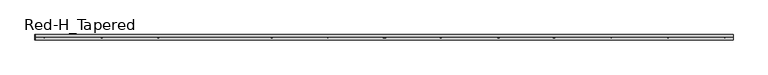
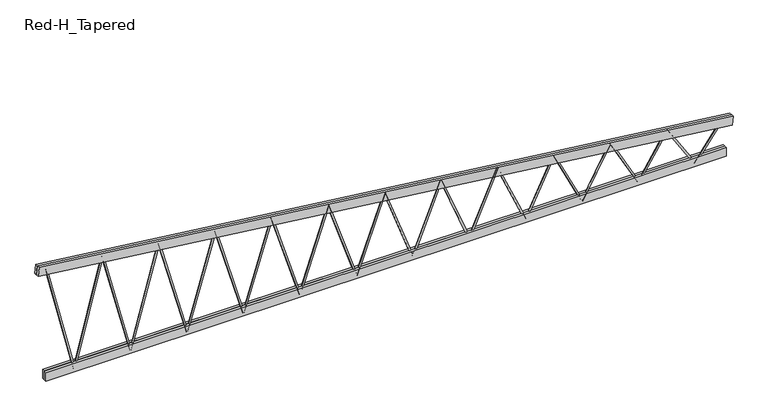
"""IFC4 building model written with IfcOpenShell, lengths in millimetres: beam geometry, Construction_Frames_RedBuilt_Openweb_Red-H_Tapered : Red-H_Tapered."""

from ifc_helpers import new_model, si_unit, point, frame, origin, origin_2d, place, context, project, spatial, polyline, circle_curve, trimmed, segment, composite_curve, outline, extrude, source, transform, mapped, element, save


def red_h_tapered_3554e35e(model_context):
    return source(origin(), model_context, "Body", "SweptSolid", [
        extrude(outline(composite_curve([segment(trimmed(circle_curve(origin_2d(), 12.7), [point((0.0, -12.7))], [point((0.0, 12.7))], False, "CARTESIAN"), True, "CONTINUOUS"), segment(trimmed(circle_curve(origin_2d(), 12.7), [point((0.0, 12.7))], [point((0.0, -12.7))], False, "CARTESIAN"), True, "CONTINUOUS")], self_intersect=False)), frame((-430.2126756, 0.0, -367.0101562), z_axis=(-0.31873146739711766, 0.0, 0.9478450567950861), x_axis=(0.0, -1.0, 0.0)), (0.0, 0.0, 1.0), 1349.7653027),
        extrude(outline(composite_curve([segment(trimmed(circle_curve(origin_2d(), 12.7), [point((0.0, 12.7))], [point((0.0, -12.7))], False, "CARTESIAN"), True, "CONTINUOUS"), segment(trimmed(circle_curve(origin_2d(), 12.7), [point((0.0, -12.7))], [point((0.0, 12.7))], False, "CARTESIAN"), True, "CONTINUOUS")], self_intersect=False)), frame((-1290.6380267, 0.0, -367.0101562), z_axis=(0.3187314673971197, 0.0, 0.9478450567950856), x_axis=(0.0, -1.0, 0.0)), (0.0, 0.0, 1.0), 1349.7653027),
        extrude(outline(composite_curve([segment(trimmed(circle_curve(origin_2d(), 12.7), [point((0.0, -12.7))], [point((0.0, 12.7))], False, "CARTESIAN"), True, "CONTINUOUS"), segment(trimmed(circle_curve(origin_2d(), 12.7), [point((0.0, 12.7))], [point((0.0, -12.7))], False, "CARTESIAN"), True, "CONTINUOUS")], self_intersect=False)), frame((-1290.6380267, 0.0, -367.0101562), z_axis=(-0.2978811940467248, 0.0, 0.954602951091865), x_axis=(0.0, -1.0, 0.0)), (0.0, 0.0, 1.0), 1444.2424838),
        extrude(outline(composite_curve([segment(trimmed(circle_curve(origin_2d(), 12.7), [point((0.0, -12.6999999))], [point((0.0, 12.7))], False, "CARTESIAN"), True, "CONTINUOUS"), segment(trimmed(circle_curve(origin_2d(), 12.7), [point((0.0, 12.7))], [point((0.0, -12.6999999))], False, "CARTESIAN"), True, "CONTINUOUS")], self_intersect=False)), frame((-2151.0633779, 0.0, -367.0101562), z_axis=(0.29788119404672875, 0.0, 0.9546029510918638), x_axis=(0.0, -1.0, 0.0)), (0.0, 0.0, 1.0), 1444.2424838),
        extrude(outline(composite_curve([segment(trimmed(circle_curve(origin_2d(), 12.7), [point((0.0, 12.7))], [point((0.0, -12.7))], False, "CARTESIAN"), True, "CONTINUOUS"), segment(trimmed(circle_curve(origin_2d(), 12.7), [point((0.0, -12.7))], [point((0.0, 12.7))], False, "CARTESIAN"), True, "CONTINUOUS")], self_intersect=False)), frame((-2151.0633779, 0.0, -367.0101562), z_axis=(-0.27948080603698605, 0.0, 0.9601512792559913), x_axis=(0.0, -1.0, 0.0)), (0.0, 0.0, 1.0), 1539.3281624),
        extrude(outline(composite_curve([segment(trimmed(circle_curve(origin_2d(), 12.7), [point((0.0, -12.6999999))], [point((0.0, 12.7))], False, "CARTESIAN"), True, "CONTINUOUS"), segment(trimmed(circle_curve(origin_2d(), 12.7), [point((0.0, 12.7))], [point((0.0, -12.6999999))], False, "CARTESIAN"), True, "CONTINUOUS")], self_intersect=False)), frame((-3011.488729, 0.0, -367.0101562), z_axis=(0.2794808060369842, 0.0, 0.9601512792559919), x_axis=(0.0, -1.0, 0.0)), (0.0, 0.0, 1.0), 1539.3281624),
        extrude(outline(composite_curve([segment(trimmed(circle_curve(origin_2d(), 12.7), [point((0.0, 12.7))], [point((0.0, -12.7))], False, "CARTESIAN"), True, "CONTINUOUS"), segment(trimmed(circle_curve(origin_2d(), 12.7), [point((0.0, -12.7))], [point((0.0, 12.7))], False, "CARTESIAN"), True, "CONTINUOUS")], self_intersect=False)), frame((-3011.488729, 0.0, -367.0101562), z_axis=(-0.2631405101102769, 0.0, 0.9647575197628175), x_axis=(0.0, -1.0, 0.0)), (0.0, 0.0, 1.0), 1634.9161723),
        extrude(outline(composite_curve([segment(trimmed(circle_curve(origin_2d(), 12.7), [point((0.0, -12.7))], [point((0.0, 12.7))], False, "CARTESIAN"), True, "CONTINUOUS"), segment(trimmed(circle_curve(origin_2d(), 12.7), [point((0.0, 12.7))], [point((0.0, -12.7))], False, "CARTESIAN"), True, "CONTINUOUS")], self_intersect=False)), frame((-3871.9140801, 0.0, -367.0101562), z_axis=(0.26314051011028217, 0.0, 0.9647575197628161), x_axis=(0.0, -1.0, 0.0)), (0.0, 0.0, 1.0), 1634.9161723),
        extrude(outline(composite_curve([segment(trimmed(circle_curve(origin_2d(), 12.7), [point((0.0, 12.7))], [point((0.0, -12.7))], False, "CARTESIAN"), True, "CONTINUOUS"), segment(trimmed(circle_curve(origin_2d(), 12.7), [point((0.0, -12.7))], [point((0.0, 12.7))], False, "CARTESIAN"), True, "CONTINUOUS")], self_intersect=False)), frame((-3871.9140801, 0.0, -367.0101562), z_axis=(-0.2485451996014145, 0.0, 0.9686202990620696), x_axis=(0.0, -1.0, 0.0)), (0.0, 0.0, 1.0), 1730.9232939),
        extrude(outline(composite_curve([segment(trimmed(circle_curve(origin_2d(), 12.7), [point((0.0, -12.7))], [point((0.0, 12.7))], False, "CARTESIAN"), True, "CONTINUOUS"), segment(trimmed(circle_curve(origin_2d(), 12.7), [point((0.0, 12.7))], [point((0.0, -12.7))], False, "CARTESIAN"), True, "CONTINUOUS")], self_intersect=False)), frame((-4732.3394313, 0.0, -367.0101562), z_axis=(0.24854519960141414, 0.0, 0.9686202990620696), x_axis=(0.0, -1.0, 0.0)), (0.0, 0.0, 1.0), 1730.9232939),
        extrude(outline(composite_curve([segment(trimmed(circle_curve(origin_2d(), 12.7), [point((0.0, 12.7))], [point((0.0, -12.7))], False, "CARTESIAN"), True, "CONTINUOUS"), segment(trimmed(circle_curve(origin_2d(), 12.7), [point((0.0, -12.7))], [point((0.0, 12.7))], False, "CARTESIAN"), True, "CONTINUOUS")], self_intersect=False)), frame((-4732.3394313, 0.0, -367.0101562), z_axis=(-0.2354383889559608, 0.0, 0.9718892761039303), x_axis=(0.0, -1.0, 0.0)), (0.0, 0.0, 1.0), 1827.2834667),
        extrude(outline(composite_curve([segment(trimmed(circle_curve(origin_2d(), 12.7), [point((0.0, 12.7000001))], [point((0.0, -12.7))], False, "CARTESIAN"), True, "CONTINUOUS"), segment(trimmed(circle_curve(origin_2d(), 12.7), [point((0.0, -12.7))], [point((0.0, 12.7000001))], False, "CARTESIAN"), True, "CONTINUOUS")], self_intersect=False)), frame((4732.3394313, 0.0, -367.0101562), z_axis=(0.5929752551345785, 0.0, 0.8052206820481461), x_axis=(0.0, -1.0, 0.0)), (0.0, 0.0, 1.0), 725.5153935),
        extrude(outline(composite_curve([segment(trimmed(circle_curve(origin_2d(), 12.7), [point((0.0, -12.7))], [point((0.0, 12.6999999))], False, "CARTESIAN"), True, "CONTINUOUS"), segment(trimmed(circle_curve(origin_2d(), 12.7), [point((0.0, 12.6999999))], [point((0.0, -12.7))], False, "CARTESIAN"), True, "CONTINUOUS")], self_intersect=False)), frame((4732.3394313, 0.0, -367.0101562), z_axis=(-0.5326844059976107, 0.0, 0.8463139627862539), x_axis=(0.0, -1.0, 0.0)), (0.0, 0.0, 1.0), 807.6314432),
        extrude(outline(composite_curve([segment(trimmed(circle_curve(origin_2d(), 12.7), [point((0.0, 12.7000001))], [point((0.0, -12.6999999))], False, "CARTESIAN"), True, "CONTINUOUS"), segment(trimmed(circle_curve(origin_2d(), 12.7), [point((0.0, -12.6999999))], [point((0.0, 12.7000001))], False, "CARTESIAN"), True, "CONTINUOUS")], self_intersect=False)), frame((3871.9140801, 0.0, -367.0101562), z_axis=(0.5326844059976091, 0.0, 0.8463139627862549), x_axis=(0.0, -1.0, 0.0)), (0.0, 0.0, 1.0), 807.6314432),
        extrude(outline(composite_curve([segment(trimmed(circle_curve(origin_2d(), 12.7), [point((0.0, -12.7))], [point((0.0, 12.7))], False, "CARTESIAN"), True, "CONTINUOUS"), segment(trimmed(circle_curve(origin_2d(), 12.7), [point((0.0, 12.7))], [point((0.0, -12.7))], False, "CARTESIAN"), True, "CONTINUOUS")], self_intersect=False)), frame((3871.9140801, 0.0, -367.0101562), z_axis=(-0.4816281502046464, 0.0, 0.8763756756839219), x_axis=(0.0, -1.0, 0.0)), (0.0, 0.0, 1.0), 893.2465334),
        extrude(outline(composite_curve([segment(trimmed(circle_curve(origin_2d(), 12.7), [point((0.0, 12.7000001))], [point((0.0, -12.7))], False, "CARTESIAN"), True, "CONTINUOUS"), segment(trimmed(circle_curve(origin_2d(), 12.7), [point((0.0, -12.7))], [point((0.0, 12.7000001))], False, "CARTESIAN"), True, "CONTINUOUS")], self_intersect=False)), frame((3011.488729, 0.0, -367.0101562), z_axis=(0.48162815020464855, 0.0, 0.8763756756839207), x_axis=(0.0, -1.0, 0.0)), (0.0, 0.0, 1.0), 893.2465334),
        extrude(outline(composite_curve([segment(trimmed(circle_curve(origin_2d(), 12.7), [point((0.0, -12.7))], [point((0.0, 12.7))], False, "CARTESIAN"), True, "CONTINUOUS"), segment(trimmed(circle_curve(origin_2d(), 12.7), [point((0.0, 12.7))], [point((0.0, -12.7))], False, "CARTESIAN"), True, "CONTINUOUS")], self_intersect=False)), frame((3011.488729, 0.0, -367.0101562), z_axis=(-0.43834601558162534, 0.0, 0.8988063031731105), x_axis=(0.0, -1.0, 0.0)), (0.0, 0.0, 1.0), 981.4453885),
        extrude(outline(composite_curve([segment(trimmed(circle_curve(origin_2d(), 12.7), [point((0.0, 12.7))], [point((0.0, -12.7))], False, "CARTESIAN"), True, "CONTINUOUS"), segment(trimmed(circle_curve(origin_2d(), 12.7), [point((0.0, -12.7))], [point((0.0, 12.7))], False, "CARTESIAN"), True, "CONTINUOUS")], self_intersect=False)), frame((2151.0633779, 0.0, -367.0101562), z_axis=(0.43834601558162795, 0.0, 0.8988063031731094), x_axis=(0.0, -1.0, 0.0)), (0.0, 0.0, 1.0), 981.4453885),
        extrude(outline(composite_curve([segment(trimmed(circle_curve(origin_2d(), 12.7), [point((0.0, -12.7))], [point((0.0, 12.6999999))], False, "CARTESIAN"), True, "CONTINUOUS"), segment(trimmed(circle_curve(origin_2d(), 12.7), [point((0.0, 12.6999999))], [point((0.0, -12.7))], False, "CARTESIAN"), True, "CONTINUOUS")], self_intersect=False)), frame((2151.0633779, 0.0, -367.0101562), z_axis=(-0.4014712611706427, 0.0, 0.9158716211642621), x_axis=(0.0, -1.0, 0.0)), (0.0, 0.0, 1.0), 1071.5902162),
        extrude(outline(composite_curve([segment(trimmed(circle_curve(origin_2d(), 12.7), [point((0.0, 12.7))], [point((0.0, -12.7))], False, "CARTESIAN"), True, "CONTINUOUS"), segment(trimmed(circle_curve(origin_2d(), 12.7), [point((0.0, -12.7))], [point((0.0, 12.7))], False, "CARTESIAN"), True, "CONTINUOUS")], self_intersect=False)), frame((1290.6380267, 0.0, -367.0101562), z_axis=(0.4014712611706487, 0.0, 0.9158716211642596), x_axis=(0.0, -1.0, 0.0)), (0.0, 0.0, 1.0), 1071.5902162),
        extrude(outline(composite_curve([segment(trimmed(circle_curve(origin_2d(), 12.7), [point((0.0, -12.7))], [point((0.0, 12.7))], False, "CARTESIAN"), True, "CONTINUOUS"), segment(trimmed(circle_curve(origin_2d(), 12.7), [point((0.0, 12.7))], [point((0.0, -12.7))], False, "CARTESIAN"), True, "CONTINUOUS")], self_intersect=False)), frame((1290.6380267, 0.0, -367.0101562), z_axis=(-0.36984358980866666, 0.0, 0.9290940313431353), x_axis=(0.0, -1.0, 0.0)), (0.0, 0.0, 1.0), 1163.228693),
        extrude(outline(composite_curve([segment(trimmed(circle_curve(origin_2d(), 12.7), [point((0.0, 12.7))], [point((0.0, -12.7))], False, "CARTESIAN"), True, "CONTINUOUS"), segment(trimmed(circle_curve(origin_2d(), 12.7), [point((0.0, -12.7))], [point((0.0, 12.7))], False, "CARTESIAN"), True, "CONTINUOUS")], self_intersect=False)), frame((430.2126756, 0.0, -367.0101562), z_axis=(0.3698435898086691, 0.0, 0.9290940313431343), x_axis=(0.0, -1.0, 0.0)), (0.0, 0.0, 1.0), 1163.228693),
        extrude(outline(composite_curve([segment(trimmed(circle_curve(origin_2d(), 12.7), [point((0.0, -12.7))], [point((0.0, 12.7))], False, "CARTESIAN"), True, "CONTINUOUS"), segment(trimmed(circle_curve(origin_2d(), 12.7), [point((0.0, 12.7))], [point((0.0, -12.7))], False, "CARTESIAN"), True, "CONTINUOUS")], self_intersect=False)), frame((430.2126756, 0.0, -367.0101562), z_axis=(-0.3425167606493955, 0.0, 0.9395117182208239), x_axis=(0.0, -1.0, 0.0)), (0.0, 0.0, 1.0), 1256.0339376),
        extrude(outline(composite_curve([segment(trimmed(circle_curve(origin_2d(), 12.7), [point((0.0, 12.7))], [point((0.0, -12.7))], False, "CARTESIAN"), True, "CONTINUOUS"), segment(trimmed(circle_curve(origin_2d(), 12.7), [point((0.0, -12.7))], [point((0.0, 12.7))], False, "CARTESIAN"), True, "CONTINUOUS")], self_intersect=False)), frame((-430.2126756, 0.0, -367.0101562), z_axis=(0.3425167606493624, 0.0, 0.9395117182208359), x_axis=(0.0, -1.0, 0.0)), (0.0, 0.0, 1.0), 1256.0339376),
        extrude(outline(polyline([(-5187.9521069, -41.275), (-5187.9521069, -3.175), (5187.9521069, -3.175), (5187.9521069, -41.275), (-5187.9521069, -41.275)])), frame((0.0, 0.0, -386.0601562), z_axis=(0.0, 0.0, 1.0), x_axis=(1.0, 0.0, 0.0)), (0.0, 0.0, 1.0), 139.7),
        extrude(outline(polyline([(-5187.9521069, 3.175), (-5187.9521069, 41.275), (5187.9521069, 41.275), (5187.9521069, 3.175), (-5187.9521069, 3.175)])), frame((0.0, 0.0, -386.0601562), z_axis=(0.0, 0.0, 1.0), x_axis=(1.0, 0.0, 0.0)), (0.0, 0.0, 1.0), 139.7),
        extrude(outline(polyline([(0.0, -38.1), (0.0, 0.0), (10654.1188147, 0.0), (10654.1188147, -38.1), (0.0, -38.1)])), frame((-5306.1006487, -3.175, 1346.8859577), z_axis=(0.11845770841726733, 0.0, 0.9929590985113786), x_axis=(0.9929590985113786, 0.0, -0.11845770841726733)), (0.0, 0.0, 1.0), 139.7),
        extrude(outline(polyline([(0.0, -38.1), (0.0, 0.0), (10654.1188147, 0.0), (10654.1188147, -38.1), (0.0, -38.1)])), frame((-5306.1006487, 41.275, 1346.8859577), z_axis=(0.11845770841726733, 0.0, 0.9929590985113786), x_axis=(0.9929590985113786, 0.0, -0.11845770841726733)), (0.0, 0.0, 1.0), 139.7),
    ])


if __name__ == "__main__":
    model = new_model("IFC4")
    model_context = context("Model", 3, world=origin())
    ifc_project = project(units=[si_unit("LENGTHUNIT", "METRE", prefix="MILLI")], contexts=[model_context])
    site = spatial("IfcSite", under=ifc_project)
    building = spatial("IfcBuilding", under=site)
    placement = place(None, origin())
    red_h_tapered_shape = red_h_tapered_3554e35e(model_context)
    element("IfcBeam", 1, ObjectType="Construction_Frames_RedBuilt_Openweb_Red-H_Tapered : Red-H_Tapered", at=placement, inside=building, context=model_context, shape_type="MappedRepresentation", body=[
        mapped(red_h_tapered_shape, transform((0.0, 0.0, 0.0), x_axis=(1.0, 0.0, 0.0), y_axis=(0.0, 1.0, 0.0), z_axis=(0.0, 0.0, 1.0))),
    ])
    save(model, "model.ifc")

# Revit data of these elements
# Type "Construction_Frames_RedBuilt_Openweb_Red-H_Tapered : Red-H_Tapered"
#   Youtube clip = ""
#   Weight Net (Kg) = "0"
#   Webs = "Up to 2\" diameter tubular steel"
#   Uniformat II Description = ""
#   Uniformat II Code = ""
#   Uniclass 2015 Name = "Softwood trusses"
#   Uniclass 2015 Code = "Pr_20_85_90_81"
#   Uniclass 2.0 Description = "Structural Framing Systems"
#   Uniclass 2.0 Code = "SS-15-10-75"
#   Uniclass 1.4 Description = "Trusses"
#   Uniclass 1.4 Code = "L3523"
#   UNSPSC Code = "30103606"
#   Technical description = "http://www.redbuilt.com/reference/literature-and-other-resources"
#   Region South America = "None"
#   Region Oceania = "None"
#   Region North America = "US"
#   Region Middle East = "None"
#   Region Europe = "None"
#   Region Asia = "None"
#   Region Antarctica = "None"
#   Region Africa = "None"
#   QR code = "http://bimobject.com/redbuilt/product/redbuilt-0003"
#   Product url = "http://www.redbuilt.com/products/default.aspx?id=2"
#   Product group = "Wood Trusses"
#   Product family = "Construction"
#   Product data url = "https://bimobject.com/redbuilt/product/redbuilt-0003"
#   Product certification = ""
#   Product SKU = "redbuilt-0003"
#   Product Page URL = "http://www.redbuilt.com/commercial-systems/red-m-red-h-open-web-trusses"
#   Product Guid = "2c5793f2-6ffb-4665-b825-cf90c048e711"
#   Product Documentation Link = "http://www.redbuilt.com/documents/OW_Guide_2017_07_LowRes_wLinks.pdf"
#   OmniClass Description = "Wood Trusses"
#   OmniClass Code = "23-13 35 19 13 17"
#   NBS Reference Description = ""
#   NBS Reference Code = ""
#   Material secondary = "Steel"
#   Material main = "Wood"
#   Masterformat 2014 Description = "Metal-Web Wood Joists"
#   Masterformat 2014 Code = "06 17 36"
#   Manufacturer name = "RedBuilt"
#   Manufacturer country = "United States"
#   Installation instructions = "http://www.redbuilt.com/documents/Installation_Sheets_Open-Web.pdf"
#   IFC Classification = ""
#   EAN code = ""
#   Design country = "United States"
#   Product Information = "http://redbuilt.com/products/default.aspx?id=2"
#   Model = "Red-H-Tapered"
#   Manufacturer URL = "http://redbuilt.com/"
#   Manufacturer = "RedBuilt™"
#   Description = "Open Web Truss"
#   Date of publishing = "8/17/2010"
#   Contact us = "http://redbuilt.com/contact/"
#   Chords = "Double 1½\" x 5½\" MSR lumber"
#   COBIe Type Category = ""
#   Brand url = "http://www.redbuilt.com"
#   BIMobject main category code = "construction"
#   BIMobject main category = "Construction"
#   BIMobject category code = "construction-frames-trusses"
#   BIMobject category = "Frames & Trusses"
#   Web Radius = 0' - 0 1/2"
#   Web Layout Offset Start [instance default] = 0' - 5"
#   Web Layout Offset End [instance default] = 0' - 5"
#   Web Diameter = 0' - 1"
#   TotalLength [instance default] = 20' - 0"
#   Span Minimum = 4' - 0"
#   Span Maximum = 70' - 0"
#   Span Limit [instance default] = 20' - 0"
#   Nominal width = 0' - 0"
#   Nominal height = 0' - 0"
#   Inner Depth Top [instance default] = 0' - 2.76372"
#   Depth Start [instance default] = 6' - 0"
#   Top Chord Length [instance default] = 20' - 1.19701"
#   TC Extension Start Aux [instance default] = 0' - 0"
#   TC Extension End Aux [instance default] = 0' - 0"
#   T-B Chord Length Difference L [instance default] = 0' - 4"
#   T-B Chord Length Difference [instance default] = 0' - 4"
#   Height 2 [instance default] = 6' - 0"
#   Depth Minimum at Wall = 2' - 0"
#   Depth Maximum at Wall = 6' - 0"
#   Depth Lower End [instance default] = 2' - 0"
#   Depth Higher End [instance default] = 6' - 0"
#   Depth End [instance default] = 2' - 0"
#   Depth 2 [instance default] = 2' - 0"
#   Chord Width = 0' - 3 1/4"
#   Chord Thickness = 0' - 1 1/2"
#   Chord Depth = 0' - 5 1/2"
#   Offset Start [instance default] = 0' - 0"
#   TC Extension Start [instance default] = 0' - 0"
#   End Panel = 0' - 5"
#   Offset End [instance default] = 0' - 0"
#   TC Extension End [instance default] = 0' - 0"
#   Length [instance default] = 20' - 0"
#   Angle [instance default] = 5.71059°
#   Span Limit Warning [instance default] = no
#   Edition number = 1
#   Top Bearing Start [instance default] = yes
#   Top Bearing End [instance default] = yes
#   Bottom Bearing Start [instance default] = no
#   Bottom Bearing End [instance default] = no
#   8 Panels [instance default] = yes
#   16 Panels [instance default] = no
#   12 Panels [instance default] = no
#   Web Material = RedBuilt-Steel, Galvanized
#   Clip Material = RedBuilt-Steel, Galvanized
#   Chords Material = RedBuilt-MSR
#   URL = ""
#   Assembly Code = ""
# Element 1 (IfcBeam, "Construction_Frames_RedBuilt_Openweb_Red-H_Tapered : Red-H_Tapered")
#   TotalLength = 34' - 8.50017"
#   Span Limit = 34' - 8.50017"
#   Inner Depth Top = 0' - 2.7695"
#   Top Chord Length = 34' - 11.4535"
#   Depth 2 = 4' - 1 11/16"
#   Angle = 6.8031°
#   8 Panels = no
#   12 Panels = yes
#   Materials on its faces: "RedBuilt-Steel, Galvanized", "RedBuilt-MSR"
# Materials
#   "RedBuilt-Steel, Galvanized": class "Metal", colour RGB 164 172 176, transparency 0, Manufacturer = "RedBuilt. LLC", Comments = "Openweb Metal Web", URL = "http://www.redbuilt.com/", Description = "Galvanized steel", Cost = 0
#   "RedBuilt-MSR": class "Wood", colour RGB 213 182 136, transparency 0, Manufacturer = "RedBuilt, LLC", URL = "http://www.redbuilt.com/", Cost = 0
